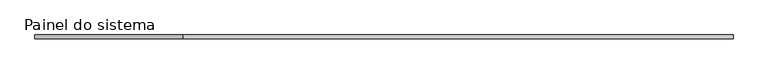
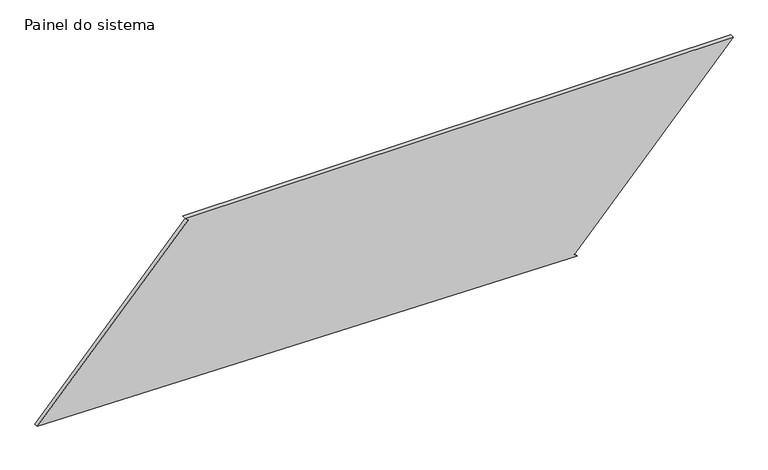
"""IFC4 building model written with IfcOpenShell, lengths in millimetres: plate geometry, Painel do sistema : Envidraçado."""

from ifc_helpers import new_model, si_unit, frame, origin, place, context, project, spatial, polyline, outline, extrude, source, transform, mapped, element, save


def painel_do_sistema_33047bde(model_context):
    return source(origin(), model_context, "Body", "SweptSolid", [
        extrude(outline(polyline([(0.0, 1207.9477923), (16.8339598, 1189.4648867), (1113.6289487, 2188.4097083), (1113.6289487, -1257.5162226), (1096.7949889, -1239.0333171), (54.4238329, -2188.4097083), (0.0, 1207.9477923)])), frame((0.0, 24.5, 0.0), z_axis=(0.0, 1.0, 0.0), x_axis=(0.0, 0.0, 1.0)), (0.0, 0.0, 1.0), 25.0),
    ])


if __name__ == "__main__":
    model = new_model("IFC4")
    model_context = context("Model", 3, world=origin())
    ifc_project = project(units=[si_unit("LENGTHUNIT", "METRE", prefix="MILLI")], contexts=[model_context])
    site = spatial("IfcSite", under=ifc_project)
    building = spatial("IfcBuilding", under=site)
    placement = place(None, origin())
    painel_do_sistema_shape = painel_do_sistema_33047bde(model_context)
    element("IfcPlate", 1, ObjectType="Painel do sistema : Envidraçado", at=placement, inside=building, context=model_context, shape_type="MappedRepresentation", body=[
        mapped(painel_do_sistema_shape, transform((0.0, 0.0, 0.0), x_axis=(1.0, 0.0, 0.0), y_axis=(0.0, 1.0, 0.0), z_axis=(0.0, 0.0, 1.0))),
    ])
    save(model, "model.ifc")

# Revit data of these elements
# Type "Painel do sistema : Envidraçado"
#   Construction Type Id = "GSP4R"
#   Analytic Construction = "Vidraça única Pilkington 1/8 pol"
#   Visual Light Transmittance = 0.9
#   Solar Heat Gain Coefficient = 0.86
#   Heat Transfer Coefficient (U) = 6.7069 W/(m²·K)
# Element 1 (IfcPlate, "Painel do sistema : Envidraçado")
#   Materials on its faces: "Vidro"
# Materials
#   "Vidro": class "Vidro", colour RGB 0 128 192, transparency 0.9, Description = "Vidro de sílica", Cost = 0
